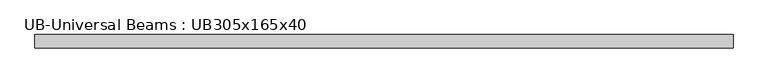
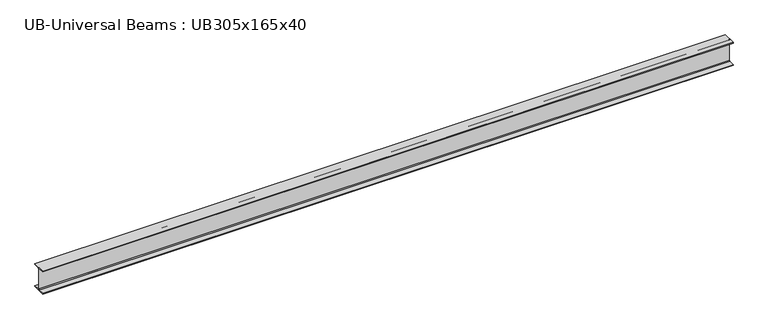
"""IFC4 building model written with IfcOpenShell, lengths in millimetres: beam geometry, UB-Universal Beams : UB305x165x40."""

from ifc_helpers import new_model, si_unit, point, frame, frame_2d, origin, place, context, project, spatial, polyline, circle_curve, trimmed, segment, composite_curve, outline, extrude, source, transform, mapped, element, save


def ub_universal_beams_ub305x165x40_6dcc7521(model_context):
    return source(origin(), model_context, "Body", "SweptSolid", [
        extrude(outline(composite_curve([segment(polyline([(82.5, -141.5), (82.5, -151.7), (-82.5, -151.7), (-82.5, -141.5), (-11.9, -141.5)]), True, "CONTINUOUS"), segment(trimmed(circle_curve(frame_2d((-11.9, -132.6)), 8.9), [point((-11.9, -141.5))], [point((-3.0, -132.6))], True, "CARTESIAN"), True, "CONTINUOUS"), segment(polyline([(-3.0, -132.6), (-3.0, 132.6)]), True, "CONTINUOUS"), segment(trimmed(circle_curve(frame_2d((-11.9, 132.6)), 8.9), [point((-3.0, 132.6))], [point((-11.9, 141.5))], True, "CARTESIAN"), True, "CONTINUOUS"), segment(polyline([(-11.9, 141.5), (-82.5, 141.5), (-82.5, 151.7), (82.5, 151.7), (82.5, 141.5), (11.9, 141.5)]), True, "CONTINUOUS"), segment(trimmed(circle_curve(frame_2d((11.9, 132.6)), 8.9), [point((11.9, 141.5))], [point((3.0, 132.6))], True, "CARTESIAN"), True, "CONTINUOUS"), segment(polyline([(3.0, 132.6), (3.0, -132.6)]), True, "CONTINUOUS"), segment(trimmed(circle_curve(frame_2d((11.9, -132.6)), 8.9), [point((3.0, -132.6))], [point((11.9, -141.5))], True, "CARTESIAN"), True, "CONTINUOUS"), segment(polyline([(11.9, -141.5), (82.5, -141.5)]), True, "CONTINUOUS")], self_intersect=False)), frame((-4333.3, 0.0, 0.0), z_axis=(1.0, 0.0, 0.0), x_axis=(0.0, 1.0, 0.0)), (0.0, 0.0, 1.0), 8666.6),
    ])


if __name__ == "__main__":
    model = new_model("IFC4")
    model_context = context("Model", 3, world=origin())
    ifc_project = project(units=[si_unit("LENGTHUNIT", "METRE", prefix="MILLI")], contexts=[model_context])
    site = spatial("IfcSite", under=ifc_project)
    building = spatial("IfcBuilding", under=site)
    placement = place(None, origin())
    ub_universal_beams_ub305x165x40_shape = ub_universal_beams_ub305x165x40_6dcc7521(model_context)
    element("IfcBeam", 1, ObjectType="UB-Universal Beams : UB305x165x40", at=placement, inside=building, context=model_context, shape_type="MappedRepresentation", body=[
        mapped(ub_universal_beams_ub305x165x40_shape, transform((0.0, 0.0, 0.0), x_axis=(1.0, 0.0, 0.0), y_axis=(0.0, 1.0, 0.0), z_axis=(0.0, 0.0, 1.0))),
    ])
    save(model, "model.ifc")

# Revit data of these elements
# Type "UB-Universal Beams : UB305x165x40"
#   Section Name Key = "UB305X165X40"
#   Width = 16.5 cm
#   Web Thickness = 0.6 cm
#   Web Fillet = 0.89 cm
#   Warping Constant = 164000.0 cm⁶
#   Torsional Moment of Inertia = 14.70 cm⁴
#   Section Area = 51.3 cm²
#   Plastic Modulus weak axis = 142.0 cm³
#   Plastic Modulus strong axis = 623.0 cm³
#   Nominal Weight = 40.2999 kgf/m
#   Moment of Inertia weak axis = 764.00 cm⁴
#   Moment of Inertia strong axis = 8503.00 cm⁴
#   Height = 30.34 cm
#   Flange Thickness = 1.02 cm
#   Elastic Modulus weak axis = 92.6 cm³
#   Elastic Modulus strong axis = 560.0 cm³
#   Centroid Vertical = 15.17 cm
#   Centroid Horizontal = 8.25 cm
#   Bolt Spacing = 9.0 cm
#   Length [instance default] = 1500 mm
#   Structural Material [instance default] = Metal - Steel 43-275
#   Type Comments = ""
#   Assembly Code = ""
# Element 1 (IfcBeam, "UB-Universal Beams : UB305x165x40")
#   Materials on its faces: "Metal - Steel 43-275"
# Materials
#   "Metal - Steel 43-275": class "Metal", colour RGB 247 247 247, transparency 0, Cost = 0
